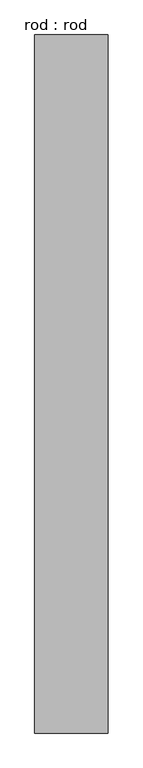
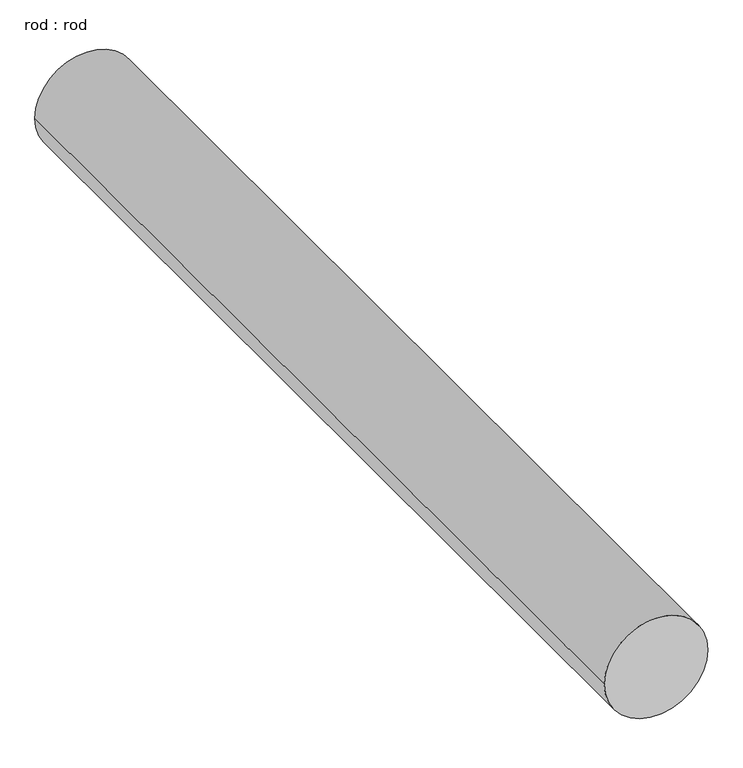
"""IFC4 building model written with IfcOpenShell, lengths in millimetres: proxy geometry, rod : rod."""

from ifc_helpers import new_model, si_unit, point, frame, frame_2d, origin, place, context, project, spatial, circle_curve, trimmed, segment, composite_curve, outline, extrude, source, transform, mapped, element, save


def rod_rod_96170eaf(model_context):
    return source(origin(), model_context, "Body", "SweptSolid", [
        extrude(outline(composite_curve([segment(trimmed(circle_curve(frame_2d((0.0108462, 0.0)), 200.0), [point((0.0108462, 200.0))], [point((0.0108462, -200.0))], False, "CARTESIAN"), True, "CONTINUOUS"), segment(trimmed(circle_curve(frame_2d((0.0108462, 0.0)), 200.0), [point((0.0108462, -200.0))], [point((0.0108462, 200.0))], False, "CARTESIAN"), True, "CONTINUOUS")], self_intersect=False)), frame((0.0, 2185.6661735, 0.0), z_axis=(0.0, 1.0, 0.0), x_axis=(0.0, 0.0, 1.0)), (0.0, 0.0, 1.0), 3814.1248837),
    ])


if __name__ == "__main__":
    model = new_model("IFC4")
    model_context = context("Model", 3, world=origin())
    ifc_project = project(units=[si_unit("LENGTHUNIT", "METRE", prefix="MILLI")], contexts=[model_context])
    site = spatial("IfcSite", under=ifc_project)
    building = spatial("IfcBuilding", under=site)
    placement = place(None, origin())
    rod_rod_shape = rod_rod_96170eaf(model_context)
    element("IfcBuildingElementProxy", 1, Name="rod : rod", ObjectType="rod : rod", at=placement, inside=building, context=model_context, shape_type="MappedRepresentation", body=[
        mapped(rod_rod_shape, transform((0.0, 0.0, 0.0), x_axis=(1.0, 0.0, 0.0), y_axis=(0.0, 1.0, 0.0), z_axis=(0.0, 0.0, 1.0))),
    ])
    save(model, "model.ifc")

# Revit data of these elements
# Type "rod : rod"
#   Default Elevation = 0
